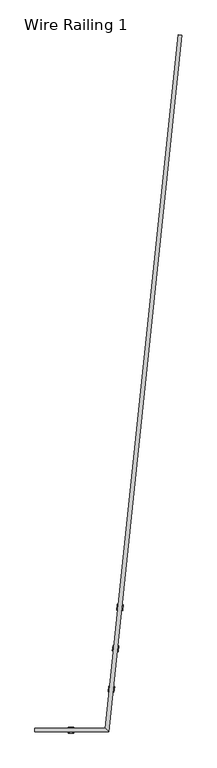
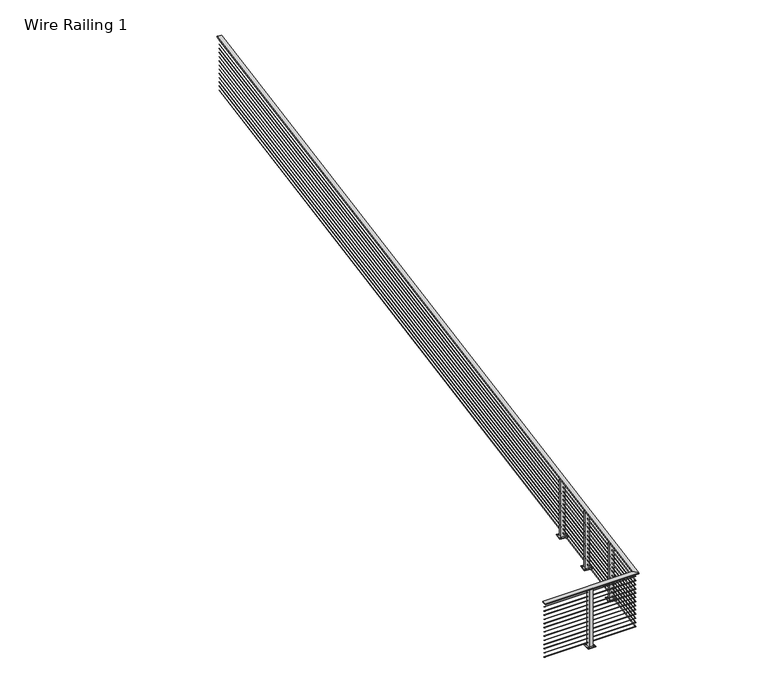
"""IFC4 building model written with IfcOpenShell, lengths in millimetres: railing geometry, Wire Railing 1."""

from ifc_helpers import new_model, si_unit, point, frame, frame_2d, origin, place, context, project, spatial, polyline, circle_curve, ellipse_curve, trimmed, segment, composite_curve, outline, extrude, faceted_brep, source, transform, mapped, element, save
from ifc_brep_helpers import plane_surface, cylinder_surface, advanced_brep


def wire_railing_1_9c637a7e(model_context):
    return source(origin(), model_context, "Body", "SolidModel", [
        faceted_brep([(32149.4090378, 25546.7031612, 267462.0), (32149.4090378, 25622.9031612, 267462.0), (32149.4090378, 25622.9031612, 267442.95), (32149.4090378, 25546.7031612, 267442.95), (33761.2935907, 25546.7031612, 267462.0), (33692.6828025, 25622.9031612, 267462.0), (33692.6828025, 25622.9031612, 267442.95), (33761.2935907, 25546.7031612, 267442.95), (35362.5021796, 40781.1852433, 267462.0), (35362.5021796, 40781.1852433, 267442.95), (35286.7196112, 40789.1503122, 267442.95), (35286.7196112, 40789.1503122, 267462.0)], [[[0, 1, 2, 3]], [[4, 5, 1, 0]], [[5, 6, 2, 1]], [[6, 7, 3, 2]], [[7, 4, 0, 3]], [[8, 9, 10, 11]], [[9, 8, 4, 7]], [[10, 9, 7, 6]], [[11, 10, 6, 5]], [[8, 11, 5, 4]]]),
        advanced_brep(
        [(32149.4090378, 25587.1844112, 267383.41875), (32149.4090378, 25582.4219112, 267383.41875), (33724.8441095, 25587.1844112, 267383.41875), (33729.1322837, 25582.4219112, 267383.41875), (35322.2426901, 40785.4166861, 267383.41875), (35326.9791007, 40784.9188693, 267383.41875)],
        [
            (0, 1, circle_curve(frame((32149.4090378, 25584.8031612, 267383.41875), z_axis=(-1.0, 0.0, 0.0), x_axis=(0.0, -1.0, 0.0)), 2.38125)),
            (1, 0, circle_curve(frame((32149.4090378, 25584.8031612, 267383.41875), z_axis=(-1.0, 0.0, 0.0), x_axis=(0.0, -1.0, 0.0)), 2.38125)),
            (2, 3, ellipse_curve(frame((33726.9881966, 25584.8031612, 267383.41875), z_axis=(-0.7431448254773928, -0.66913060635886, 0.0), x_axis=(0.6691306063588597, -0.7431448254773928, 0.0)), 3.2042879, 2.38125)),
            (3, 1),
            (0, 2),
            (3, 2, ellipse_curve(frame((33726.9881966, 25584.8031612, 267383.41875), z_axis=(-0.7431448254773928, -0.66913060635886, 0.0), x_axis=(0.6691306063588597, -0.7431448254773928, 0.0)), 3.2042879, 2.38125)),
            (4, 5, circle_curve(frame((35324.6108954, 40785.1677777, 267383.41875), z_axis=(0.10452846326764917, 0.9945218953682738, 0.0), x_axis=(0.9945218953682738, -0.10452846326764917, 0.0)), 2.38125)),
            (5, 4, circle_curve(frame((35324.6108954, 40785.1677777, 267383.41875), z_axis=(0.10452846326764917, 0.9945218953682738, 0.0), x_axis=(0.9945218953682738, -0.10452846326764917, 0.0)), 2.38125)),
            (4, 2),
            (3, 5),
        ],
        [
            plane_surface(frame((32149.4090378, 25584.8031612, 267385.8), z_axis=(-1.0, 0.0, 0.0), x_axis=(0.0, -1.0, 0.0))),
            cylinder_surface(frame((33726.9881966, 25584.8031612, 267383.41875), z_axis=(1.0, 0.0, 0.0), x_axis=(0.0, -1.0, 0.0)), 2.38125),
            plane_surface(frame((35324.6108954, 40785.1677777, 267385.8), z_axis=(0.10452846326764917, 0.9945218953682738, 0.0), x_axis=(0.9945218953682738, -0.10452846326764917, 0.0))),
            cylinder_surface(frame((35324.6108954, 40785.1677777, 267383.41875), z_axis=(0.10452846326764917, 0.9945218953682738, 0.0), x_axis=(0.9945218953682738, -0.10452846326764917, 0.0)), 2.38125),
        ],
        [
            (0, [[1, 2]]),
            (1, [[3, 4, -1, 5]]),
            (1, [[6, -5, -2, -4]]),
            (2, [[7, 8]]),
            (3, [[-7, 9, -6, 10]]),
            (3, [[-8, -10, -3, -9]]),
        ],
    ),
        advanced_brep(
        [(32149.4090378, 25587.1844112, 267307.21875), (32149.4090378, 25582.4219112, 267307.21875), (33724.8441095, 25587.1844112, 267307.21875), (33729.1322837, 25582.4219112, 267307.21875), (35322.2426901, 40785.4166861, 267307.21875), (35326.9791007, 40784.9188693, 267307.21875)],
        [
            (0, 1, circle_curve(frame((32149.4090378, 25584.8031612, 267307.21875), z_axis=(-1.0, 0.0, 0.0), x_axis=(0.0, -1.0, 0.0)), 2.38125)),
            (1, 0, circle_curve(frame((32149.4090378, 25584.8031612, 267307.21875), z_axis=(-1.0, 0.0, 0.0), x_axis=(0.0, -1.0, 0.0)), 2.38125)),
            (2, 3, ellipse_curve(frame((33726.9881966, 25584.8031612, 267307.21875), z_axis=(-0.7431448254773928, -0.66913060635886, 0.0), x_axis=(0.6691306063588597, -0.7431448254773928, 0.0)), 3.2042879, 2.38125)),
            (3, 1),
            (0, 2),
            (3, 2, ellipse_curve(frame((33726.9881966, 25584.8031612, 267307.21875), z_axis=(-0.7431448254773928, -0.66913060635886, 0.0), x_axis=(0.6691306063588597, -0.7431448254773928, 0.0)), 3.2042879, 2.38125)),
            (4, 5, circle_curve(frame((35324.6108954, 40785.1677777, 267307.21875), z_axis=(0.10452846326764917, 0.9945218953682738, 0.0), x_axis=(0.9945218953682738, -0.10452846326764917, 0.0)), 2.38125)),
            (5, 4, circle_curve(frame((35324.6108954, 40785.1677777, 267307.21875), z_axis=(0.10452846326764917, 0.9945218953682738, 0.0), x_axis=(0.9945218953682738, -0.10452846326764917, 0.0)), 2.38125)),
            (4, 2),
            (3, 5),
        ],
        [
            plane_surface(frame((32149.4090378, 25584.8031612, 267309.6), z_axis=(-1.0, 0.0, 0.0), x_axis=(0.0, -1.0, 0.0))),
            cylinder_surface(frame((33726.9881966, 25584.8031612, 267307.21875), z_axis=(1.0, 0.0, 0.0), x_axis=(0.0, -1.0, 0.0)), 2.38125),
            plane_surface(frame((35324.6108954, 40785.1677777, 267309.6), z_axis=(0.10452846326764917, 0.9945218953682738, 0.0), x_axis=(0.9945218953682738, -0.10452846326764917, 0.0))),
            cylinder_surface(frame((35324.6108954, 40785.1677777, 267307.21875), z_axis=(0.10452846326764917, 0.9945218953682738, 0.0), x_axis=(0.9945218953682738, -0.10452846326764917, 0.0)), 2.38125),
        ],
        [
            (0, [[1, 2]]),
            (1, [[3, 4, -1, 5]]),
            (1, [[6, -5, -2, -4]]),
            (2, [[7, 8]]),
            (3, [[-7, 9, -6, 10]]),
            (3, [[-8, -10, -3, -9]]),
        ],
    ),
        advanced_brep(
        [(32149.4090378, 25587.1844112, 267231.01875), (32149.4090378, 25582.4219112, 267231.01875), (33724.8441095, 25587.1844112, 267231.01875), (33729.1322837, 25582.4219112, 267231.01875), (35322.2426901, 40785.4166861, 267231.01875), (35326.9791007, 40784.9188693, 267231.01875)],
        [
            (0, 1, circle_curve(frame((32149.4090378, 25584.8031612, 267231.01875), z_axis=(-1.0, 0.0, 0.0), x_axis=(0.0, -1.0, 0.0)), 2.38125)),
            (1, 0, circle_curve(frame((32149.4090378, 25584.8031612, 267231.01875), z_axis=(-1.0, 0.0, 0.0), x_axis=(0.0, -1.0, 0.0)), 2.38125)),
            (2, 3, ellipse_curve(frame((33726.9881966, 25584.8031612, 267231.01875), z_axis=(-0.7431448254773928, -0.66913060635886, 0.0), x_axis=(0.6691306063588597, -0.7431448254773928, 0.0)), 3.2042879, 2.38125)),
            (3, 1),
            (0, 2),
            (3, 2, ellipse_curve(frame((33726.9881966, 25584.8031612, 267231.01875), z_axis=(-0.7431448254773928, -0.66913060635886, 0.0), x_axis=(0.6691306063588597, -0.7431448254773928, 0.0)), 3.2042879, 2.38125)),
            (4, 5, circle_curve(frame((35324.6108954, 40785.1677777, 267231.01875), z_axis=(0.10452846326764917, 0.9945218953682738, 0.0), x_axis=(0.9945218953682738, -0.10452846326764917, 0.0)), 2.38125)),
            (5, 4, circle_curve(frame((35324.6108954, 40785.1677777, 267231.01875), z_axis=(0.10452846326764917, 0.9945218953682738, 0.0), x_axis=(0.9945218953682738, -0.10452846326764917, 0.0)), 2.38125)),
            (4, 2),
            (3, 5),
        ],
        [
            plane_surface(frame((32149.4090378, 25584.8031612, 267233.4), z_axis=(-1.0, 0.0, 0.0), x_axis=(0.0, -1.0, 0.0))),
            cylinder_surface(frame((33726.9881966, 25584.8031612, 267231.01875), z_axis=(1.0, 0.0, 0.0), x_axis=(0.0, -1.0, 0.0)), 2.38125),
            plane_surface(frame((35324.6108954, 40785.1677777, 267233.4), z_axis=(0.10452846326764917, 0.9945218953682738, 0.0), x_axis=(0.9945218953682738, -0.10452846326764917, 0.0))),
            cylinder_surface(frame((35324.6108954, 40785.1677777, 267231.01875), z_axis=(0.10452846326764917, 0.9945218953682738, 0.0), x_axis=(0.9945218953682738, -0.10452846326764917, 0.0)), 2.38125),
        ],
        [
            (0, [[1, 2]]),
            (1, [[3, 4, -1, 5]]),
            (1, [[6, -5, -2, -4]]),
            (2, [[7, 8]]),
            (3, [[-7, 9, -6, 10]]),
            (3, [[-8, -10, -3, -9]]),
        ],
    ),
        advanced_brep(
        [(32149.4090378, 25587.1844112, 267154.81875), (32149.4090378, 25582.4219112, 267154.81875), (33724.8441095, 25587.1844112, 267154.81875), (33729.1322837, 25582.4219112, 267154.81875), (35322.2426901, 40785.4166861, 267154.81875), (35326.9791007, 40784.9188693, 267154.81875)],
        [
            (0, 1, circle_curve(frame((32149.4090378, 25584.8031612, 267154.81875), z_axis=(-1.0, 0.0, 0.0), x_axis=(0.0, -1.0, 0.0)), 2.38125)),
            (1, 0, circle_curve(frame((32149.4090378, 25584.8031612, 267154.81875), z_axis=(-1.0, 0.0, 0.0), x_axis=(0.0, -1.0, 0.0)), 2.38125)),
            (2, 3, ellipse_curve(frame((33726.9881966, 25584.8031612, 267154.81875), z_axis=(-0.7431448254773928, -0.66913060635886, 0.0), x_axis=(0.6691306063588597, -0.7431448254773928, 0.0)), 3.2042879, 2.38125)),
            (3, 1),
            (0, 2),
            (3, 2, ellipse_curve(frame((33726.9881966, 25584.8031612, 267154.81875), z_axis=(-0.7431448254773928, -0.66913060635886, 0.0), x_axis=(0.6691306063588597, -0.7431448254773928, 0.0)), 3.2042879, 2.38125)),
            (4, 5, circle_curve(frame((35324.6108954, 40785.1677777, 267154.81875), z_axis=(0.10452846326764917, 0.9945218953682738, 0.0), x_axis=(0.9945218953682738, -0.10452846326764917, 0.0)), 2.38125)),
            (5, 4, circle_curve(frame((35324.6108954, 40785.1677777, 267154.81875), z_axis=(0.10452846326764917, 0.9945218953682738, 0.0), x_axis=(0.9945218953682738, -0.10452846326764917, 0.0)), 2.38125)),
            (4, 2),
            (3, 5),
        ],
        [
            plane_surface(frame((32149.4090378, 25584.8031612, 267157.2), z_axis=(-1.0, 0.0, 0.0), x_axis=(0.0, -1.0, 0.0))),
            cylinder_surface(frame((33726.9881966, 25584.8031612, 267154.81875), z_axis=(1.0, 0.0, 0.0), x_axis=(0.0, -1.0, 0.0)), 2.38125),
            plane_surface(frame((35324.6108954, 40785.1677777, 267157.2), z_axis=(0.10452846326764917, 0.9945218953682738, 0.0), x_axis=(0.9945218953682738, -0.10452846326764917, 0.0))),
            cylinder_surface(frame((35324.6108954, 40785.1677777, 267154.81875), z_axis=(0.10452846326764917, 0.9945218953682738, 0.0), x_axis=(0.9945218953682738, -0.10452846326764917, 0.0)), 2.38125),
        ],
        [
            (0, [[1, 2]]),
            (1, [[3, 4, -1, 5]]),
            (1, [[6, -5, -2, -4]]),
            (2, [[7, 8]]),
            (3, [[-7, 9, -6, 10]]),
            (3, [[-8, -10, -3, -9]]),
        ],
    ),
        advanced_brep(
        [(32149.4090378, 25587.1844112, 267078.61875), (32149.4090378, 25582.4219112, 267078.61875), (33724.8441095, 25587.1844112, 267078.61875), (33729.1322837, 25582.4219112, 267078.61875), (35322.2426901, 40785.4166861, 267078.61875), (35326.9791007, 40784.9188693, 267078.61875)],
        [
            (0, 1, circle_curve(frame((32149.4090378, 25584.8031612, 267078.61875), z_axis=(-1.0, 0.0, 0.0), x_axis=(0.0, -1.0, 0.0)), 2.38125)),
            (1, 0, circle_curve(frame((32149.4090378, 25584.8031612, 267078.61875), z_axis=(-1.0, 0.0, 0.0), x_axis=(0.0, -1.0, 0.0)), 2.38125)),
            (2, 3, ellipse_curve(frame((33726.9881966, 25584.8031612, 267078.61875), z_axis=(-0.7431448254773928, -0.66913060635886, 0.0), x_axis=(0.6691306063588597, -0.7431448254773928, 0.0)), 3.2042879, 2.38125)),
            (3, 1),
            (0, 2),
            (3, 2, ellipse_curve(frame((33726.9881966, 25584.8031612, 267078.61875), z_axis=(-0.7431448254773928, -0.66913060635886, 0.0), x_axis=(0.6691306063588597, -0.7431448254773928, 0.0)), 3.2042879, 2.38125)),
            (4, 5, circle_curve(frame((35324.6108954, 40785.1677777, 267078.61875), z_axis=(0.10452846326764917, 0.9945218953682738, 0.0), x_axis=(0.9945218953682738, -0.10452846326764917, 0.0)), 2.38125)),
            (5, 4, circle_curve(frame((35324.6108954, 40785.1677777, 267078.61875), z_axis=(0.10452846326764917, 0.9945218953682738, 0.0), x_axis=(0.9945218953682738, -0.10452846326764917, 0.0)), 2.38125)),
            (4, 2),
            (3, 5),
        ],
        [
            plane_surface(frame((32149.4090378, 25584.8031612, 267081.0), z_axis=(-1.0, 0.0, 0.0), x_axis=(0.0, -1.0, 0.0))),
            cylinder_surface(frame((33726.9881966, 25584.8031612, 267078.61875), z_axis=(1.0, 0.0, 0.0), x_axis=(0.0, -1.0, 0.0)), 2.38125),
            plane_surface(frame((35324.6108954, 40785.1677777, 267081.0), z_axis=(0.10452846326764917, 0.9945218953682738, 0.0), x_axis=(0.9945218953682738, -0.10452846326764917, 0.0))),
            cylinder_surface(frame((35324.6108954, 40785.1677777, 267078.61875), z_axis=(0.10452846326764917, 0.9945218953682738, 0.0), x_axis=(0.9945218953682738, -0.10452846326764917, 0.0)), 2.38125),
        ],
        [
            (0, [[1, 2]]),
            (1, [[3, 4, -1, 5]]),
            (1, [[6, -5, -2, -4]]),
            (2, [[7, 8]]),
            (3, [[-7, 9, -6, 10]]),
            (3, [[-8, -10, -3, -9]]),
        ],
    ),
        advanced_brep(
        [(32149.4090378, 25587.1844112, 267002.41875), (32149.4090378, 25582.4219112, 267002.41875), (33724.8441095, 25587.1844112, 267002.41875), (33729.1322837, 25582.4219112, 267002.41875), (35322.2426901, 40785.4166861, 267002.41875), (35326.9791007, 40784.9188693, 267002.41875)],
        [
            (0, 1, circle_curve(frame((32149.4090378, 25584.8031612, 267002.41875), z_axis=(-1.0, 0.0, 0.0), x_axis=(0.0, -1.0, 0.0)), 2.38125)),
            (1, 0, circle_curve(frame((32149.4090378, 25584.8031612, 267002.41875), z_axis=(-1.0, 0.0, 0.0), x_axis=(0.0, -1.0, 0.0)), 2.38125)),
            (2, 3, ellipse_curve(frame((33726.9881966, 25584.8031612, 267002.41875), z_axis=(-0.7431448254773928, -0.66913060635886, 0.0), x_axis=(0.6691306063588597, -0.7431448254773928, 0.0)), 3.2042879, 2.38125)),
            (3, 1),
            (0, 2),
            (3, 2, ellipse_curve(frame((33726.9881966, 25584.8031612, 267002.41875), z_axis=(-0.7431448254773928, -0.66913060635886, 0.0), x_axis=(0.6691306063588597, -0.7431448254773928, 0.0)), 3.2042879, 2.38125)),
            (4, 5, circle_curve(frame((35324.6108954, 40785.1677777, 267002.41875), z_axis=(0.10452846326764917, 0.9945218953682738, 0.0), x_axis=(0.9945218953682738, -0.10452846326764917, 0.0)), 2.38125)),
            (5, 4, circle_curve(frame((35324.6108954, 40785.1677777, 267002.41875), z_axis=(0.10452846326764917, 0.9945218953682738, 0.0), x_axis=(0.9945218953682738, -0.10452846326764917, 0.0)), 2.38125)),
            (4, 2),
            (3, 5),
        ],
        [
            plane_surface(frame((32149.4090378, 25584.8031612, 267004.8), z_axis=(-1.0, 0.0, 0.0), x_axis=(0.0, -1.0, 0.0))),
            cylinder_surface(frame((33726.9881966, 25584.8031612, 267002.41875), z_axis=(1.0, 0.0, 0.0), x_axis=(0.0, -1.0, 0.0)), 2.38125),
            plane_surface(frame((35324.6108954, 40785.1677777, 267004.8), z_axis=(0.10452846326764917, 0.9945218953682738, 0.0), x_axis=(0.9945218953682738, -0.10452846326764917, 0.0))),
            cylinder_surface(frame((35324.6108954, 40785.1677777, 267002.41875), z_axis=(0.10452846326764917, 0.9945218953682738, 0.0), x_axis=(0.9945218953682738, -0.10452846326764917, 0.0)), 2.38125),
        ],
        [
            (0, [[1, 2]]),
            (1, [[3, 4, -1, 5]]),
            (1, [[6, -5, -2, -4]]),
            (2, [[7, 8]]),
            (3, [[-7, 9, -6, 10]]),
            (3, [[-8, -10, -3, -9]]),
        ],
    ),
        advanced_brep(
        [(32149.4090378, 25587.1844112, 266926.21875), (32149.4090378, 25582.4219112, 266926.21875), (33724.8441095, 25587.1844112, 266926.21875), (33729.1322837, 25582.4219112, 266926.21875), (35322.2426901, 40785.4166861, 266926.21875), (35326.9791007, 40784.9188693, 266926.21875)],
        [
            (0, 1, circle_curve(frame((32149.4090378, 25584.8031612, 266926.21875), z_axis=(-1.0, 0.0, 0.0), x_axis=(0.0, -1.0, 0.0)), 2.38125)),
            (1, 0, circle_curve(frame((32149.4090378, 25584.8031612, 266926.21875), z_axis=(-1.0, 0.0, 0.0), x_axis=(0.0, -1.0, 0.0)), 2.38125)),
            (2, 3, ellipse_curve(frame((33726.9881966, 25584.8031612, 266926.21875), z_axis=(-0.7431448254773928, -0.66913060635886, 0.0), x_axis=(0.6691306063588597, -0.7431448254773928, 0.0)), 3.2042879, 2.38125)),
            (3, 1),
            (0, 2),
            (3, 2, ellipse_curve(frame((33726.9881966, 25584.8031612, 266926.21875), z_axis=(-0.7431448254773928, -0.66913060635886, 0.0), x_axis=(0.6691306063588597, -0.7431448254773928, 0.0)), 3.2042879, 2.38125)),
            (4, 5, circle_curve(frame((35324.6108954, 40785.1677777, 266926.21875), z_axis=(0.10452846326764917, 0.9945218953682738, 0.0), x_axis=(0.9945218953682738, -0.10452846326764917, 0.0)), 2.38125)),
            (5, 4, circle_curve(frame((35324.6108954, 40785.1677777, 266926.21875), z_axis=(0.10452846326764917, 0.9945218953682738, 0.0), x_axis=(0.9945218953682738, -0.10452846326764917, 0.0)), 2.38125)),
            (4, 2),
            (3, 5),
        ],
        [
            plane_surface(frame((32149.4090378, 25584.8031612, 266928.6), z_axis=(-1.0, 0.0, 0.0), x_axis=(0.0, -1.0, 0.0))),
            cylinder_surface(frame((33726.9881966, 25584.8031612, 266926.21875), z_axis=(1.0, 0.0, 0.0), x_axis=(0.0, -1.0, 0.0)), 2.38125),
            plane_surface(frame((35324.6108954, 40785.1677777, 266928.6), z_axis=(0.10452846326764917, 0.9945218953682738, 0.0), x_axis=(0.9945218953682738, -0.10452846326764917, 0.0))),
            cylinder_surface(frame((35324.6108954, 40785.1677777, 266926.21875), z_axis=(0.10452846326764917, 0.9945218953682738, 0.0), x_axis=(0.9945218953682738, -0.10452846326764917, 0.0)), 2.38125),
        ],
        [
            (0, [[1, 2]]),
            (1, [[3, 4, -1, 5]]),
            (1, [[6, -5, -2, -4]]),
            (2, [[7, 8]]),
            (3, [[-7, 9, -6, 10]]),
            (3, [[-8, -10, -3, -9]]),
        ],
    ),
        advanced_brep(
        [(32149.4090378, 25587.1844112, 266850.01875), (32149.4090378, 25582.4219112, 266850.01875), (33724.8441095, 25587.1844112, 266850.01875), (33729.1322837, 25582.4219112, 266850.01875), (35322.2426901, 40785.4166861, 266850.01875), (35326.9791007, 40784.9188693, 266850.01875)],
        [
            (0, 1, circle_curve(frame((32149.4090378, 25584.8031612, 266850.01875), z_axis=(-1.0, 0.0, 0.0), x_axis=(0.0, -1.0, 0.0)), 2.38125)),
            (1, 0, circle_curve(frame((32149.4090378, 25584.8031612, 266850.01875), z_axis=(-1.0, 0.0, 0.0), x_axis=(0.0, -1.0, 0.0)), 2.38125)),
            (2, 3, ellipse_curve(frame((33726.9881966, 25584.8031612, 266850.01875), z_axis=(-0.7431448254773928, -0.66913060635886, 0.0), x_axis=(0.6691306063588597, -0.7431448254773928, 0.0)), 3.2042879, 2.38125)),
            (3, 1),
            (0, 2),
            (3, 2, ellipse_curve(frame((33726.9881966, 25584.8031612, 266850.01875), z_axis=(-0.7431448254773928, -0.66913060635886, 0.0), x_axis=(0.6691306063588597, -0.7431448254773928, 0.0)), 3.2042879, 2.38125)),
            (4, 5, circle_curve(frame((35324.6108954, 40785.1677777, 266850.01875), z_axis=(0.10452846326764917, 0.9945218953682738, 0.0), x_axis=(0.9945218953682738, -0.10452846326764917, 0.0)), 2.38125)),
            (5, 4, circle_curve(frame((35324.6108954, 40785.1677777, 266850.01875), z_axis=(0.10452846326764917, 0.9945218953682738, 0.0), x_axis=(0.9945218953682738, -0.10452846326764917, 0.0)), 2.38125)),
            (4, 2),
            (3, 5),
        ],
        [
            plane_surface(frame((32149.4090378, 25584.8031612, 266852.4), z_axis=(-1.0, 0.0, 0.0), x_axis=(0.0, -1.0, 0.0))),
            cylinder_surface(frame((33726.9881966, 25584.8031612, 266850.01875), z_axis=(1.0, 0.0, 0.0), x_axis=(0.0, -1.0, 0.0)), 2.38125),
            plane_surface(frame((35324.6108954, 40785.1677777, 266852.4), z_axis=(0.10452846326764917, 0.9945218953682738, 0.0), x_axis=(0.9945218953682738, -0.10452846326764917, 0.0))),
            cylinder_surface(frame((35324.6108954, 40785.1677777, 266850.01875), z_axis=(0.10452846326764917, 0.9945218953682738, 0.0), x_axis=(0.9945218953682738, -0.10452846326764917, 0.0)), 2.38125),
        ],
        [
            (0, [[1, 2]]),
            (1, [[3, 4, -1, 5]]),
            (1, [[6, -5, -2, -4]]),
            (2, [[7, 8]]),
            (3, [[-7, 9, -6, 10]]),
            (3, [[-8, -10, -3, -9]]),
        ],
    ),
        advanced_brep(
        [(32149.4090378, 25587.1844112, 266773.81875), (32149.4090378, 25582.4219112, 266773.81875), (33724.8441095, 25587.1844112, 266773.81875), (33729.1322837, 25582.4219112, 266773.81875), (35322.2426901, 40785.4166861, 266773.81875), (35326.9791007, 40784.9188693, 266773.81875)],
        [
            (0, 1, circle_curve(frame((32149.4090378, 25584.8031612, 266773.81875), z_axis=(-1.0, 0.0, 0.0), x_axis=(0.0, -1.0, 0.0)), 2.38125)),
            (1, 0, circle_curve(frame((32149.4090378, 25584.8031612, 266773.81875), z_axis=(-1.0, 0.0, 0.0), x_axis=(0.0, -1.0, 0.0)), 2.38125)),
            (2, 3, ellipse_curve(frame((33726.9881966, 25584.8031612, 266773.81875), z_axis=(-0.7431448254773928, -0.66913060635886, 0.0), x_axis=(0.6691306063588597, -0.7431448254773928, 0.0)), 3.2042879, 2.38125)),
            (3, 1),
            (0, 2),
            (3, 2, ellipse_curve(frame((33726.9881966, 25584.8031612, 266773.81875), z_axis=(-0.7431448254773928, -0.66913060635886, 0.0), x_axis=(0.6691306063588597, -0.7431448254773928, 0.0)), 3.2042879, 2.38125)),
            (4, 5, circle_curve(frame((35324.6108954, 40785.1677777, 266773.81875), z_axis=(0.10452846326764917, 0.9945218953682738, 0.0), x_axis=(0.9945218953682738, -0.10452846326764917, 0.0)), 2.38125)),
            (5, 4, circle_curve(frame((35324.6108954, 40785.1677777, 266773.81875), z_axis=(0.10452846326764917, 0.9945218953682738, 0.0), x_axis=(0.9945218953682738, -0.10452846326764917, 0.0)), 2.38125)),
            (4, 2),
            (3, 5),
        ],
        [
            plane_surface(frame((32149.4090378, 25584.8031612, 266776.2), z_axis=(-1.0, 0.0, 0.0), x_axis=(0.0, -1.0, 0.0))),
            cylinder_surface(frame((33726.9881966, 25584.8031612, 266773.81875), z_axis=(1.0, 0.0, 0.0), x_axis=(0.0, -1.0, 0.0)), 2.38125),
            plane_surface(frame((35324.6108954, 40785.1677777, 266776.2), z_axis=(0.10452846326764917, 0.9945218953682738, 0.0), x_axis=(0.9945218953682738, -0.10452846326764917, 0.0))),
            cylinder_surface(frame((35324.6108954, 40785.1677777, 266773.81875), z_axis=(0.10452846326764917, 0.9945218953682738, 0.0), x_axis=(0.9945218953682738, -0.10452846326764917, 0.0)), 2.38125),
        ],
        [
            (0, [[1, 2]]),
            (1, [[3, 4, -1, 5]]),
            (1, [[6, -5, -2, -4]]),
            (2, [[7, 8]]),
            (3, [[-7, 9, -6, 10]]),
            (3, [[-8, -10, -3, -9]]),
        ],
    ),
        advanced_brep(
        [(32149.4090378, 25587.1844112, 266697.61875), (32149.4090378, 25582.4219112, 266697.61875), (33724.8441095, 25587.1844112, 266697.61875), (33729.1322837, 25582.4219112, 266697.61875), (35322.2426901, 40785.4166861, 266697.61875), (35326.9791007, 40784.9188693, 266697.61875)],
        [
            (0, 1, circle_curve(frame((32149.4090378, 25584.8031612, 266697.61875), z_axis=(-1.0, 0.0, 0.0), x_axis=(0.0, -1.0, 0.0)), 2.38125)),
            (1, 0, circle_curve(frame((32149.4090378, 25584.8031612, 266697.61875), z_axis=(-1.0, 0.0, 0.0), x_axis=(0.0, -1.0, 0.0)), 2.38125)),
            (2, 3, ellipse_curve(frame((33726.9881966, 25584.8031612, 266697.61875), z_axis=(-0.7431448254773928, -0.66913060635886, 0.0), x_axis=(0.6691306063588597, -0.7431448254773928, 0.0)), 3.2042879, 2.38125)),
            (3, 1),
            (0, 2),
            (3, 2, ellipse_curve(frame((33726.9881966, 25584.8031612, 266697.61875), z_axis=(-0.7431448254773928, -0.66913060635886, 0.0), x_axis=(0.6691306063588597, -0.7431448254773928, 0.0)), 3.2042879, 2.38125)),
            (4, 5, circle_curve(frame((35324.6108954, 40785.1677777, 266697.61875), z_axis=(0.10452846326764917, 0.9945218953682738, 0.0), x_axis=(0.9945218953682738, -0.10452846326764917, 0.0)), 2.38125)),
            (5, 4, circle_curve(frame((35324.6108954, 40785.1677777, 266697.61875), z_axis=(0.10452846326764917, 0.9945218953682738, 0.0), x_axis=(0.9945218953682738, -0.10452846326764917, 0.0)), 2.38125)),
            (4, 2),
            (3, 5),
        ],
        [
            plane_surface(frame((32149.4090378, 25584.8031612, 266700.0), z_axis=(-1.0, 0.0, 0.0), x_axis=(0.0, -1.0, 0.0))),
            cylinder_surface(frame((33726.9881966, 25584.8031612, 266697.61875), z_axis=(1.0, 0.0, 0.0), x_axis=(0.0, -1.0, 0.0)), 2.38125),
            plane_surface(frame((35324.6108954, 40785.1677777, 266700.0), z_axis=(0.10452846326764917, 0.9945218953682738, 0.0), x_axis=(0.9945218953682738, -0.10452846326764917, 0.0))),
            cylinder_surface(frame((35324.6108954, 40785.1677777, 266697.61875), z_axis=(0.10452846326764917, 0.9945218953682738, 0.0), x_axis=(0.9945218953682738, -0.10452846326764917, 0.0)), 2.38125),
        ],
        [
            (0, [[1, 2]]),
            (1, [[3, 4, -1, 5]]),
            (1, [[6, -5, -2, -4]]),
            (2, [[7, 8]]),
            (3, [[-7, 9, -6, 10]]),
            (3, [[-8, -10, -3, -9]]),
        ],
    ),
        advanced_brep(
        [(32149.4090378, 25587.1844112, 266621.41875), (32149.4090378, 25582.4219112, 266621.41875), (33724.8441095, 25587.1844112, 266621.41875), (33729.1322837, 25582.4219112, 266621.41875), (35322.2426901, 40785.4166861, 266621.41875), (35326.9791007, 40784.9188693, 266621.41875)],
        [
            (0, 1, circle_curve(frame((32149.4090378, 25584.8031612, 266621.41875), z_axis=(-1.0, 0.0, 0.0), x_axis=(0.0, -1.0, 0.0)), 2.38125)),
            (1, 0, circle_curve(frame((32149.4090378, 25584.8031612, 266621.41875), z_axis=(-1.0, 0.0, 0.0), x_axis=(0.0, -1.0, 0.0)), 2.38125)),
            (2, 3, ellipse_curve(frame((33726.9881966, 25584.8031612, 266621.41875), z_axis=(-0.7431448254773928, -0.66913060635886, 0.0), x_axis=(0.6691306063588597, -0.7431448254773928, 0.0)), 3.2042879, 2.38125)),
            (3, 1),
            (0, 2),
            (3, 2, ellipse_curve(frame((33726.9881966, 25584.8031612, 266621.41875), z_axis=(-0.7431448254773928, -0.66913060635886, 0.0), x_axis=(0.6691306063588597, -0.7431448254773928, 0.0)), 3.2042879, 2.38125)),
            (4, 5, circle_curve(frame((35324.6108954, 40785.1677777, 266621.41875), z_axis=(0.10452846326764917, 0.9945218953682738, 0.0), x_axis=(0.9945218953682738, -0.10452846326764917, 0.0)), 2.38125)),
            (5, 4, circle_curve(frame((35324.6108954, 40785.1677777, 266621.41875), z_axis=(0.10452846326764917, 0.9945218953682738, 0.0), x_axis=(0.9945218953682738, -0.10452846326764917, 0.0)), 2.38125)),
            (4, 2),
            (3, 5),
        ],
        [
            plane_surface(frame((32149.4090378, 25584.8031612, 266623.8), z_axis=(-1.0, 0.0, 0.0), x_axis=(0.0, -1.0, 0.0))),
            cylinder_surface(frame((33726.9881966, 25584.8031612, 266621.41875), z_axis=(1.0, 0.0, 0.0), x_axis=(0.0, -1.0, 0.0)), 2.38125),
            plane_surface(frame((35324.6108954, 40785.1677777, 266623.8), z_axis=(0.10452846326764917, 0.9945218953682738, 0.0), x_axis=(0.9945218953682738, -0.10452846326764917, 0.0))),
            cylinder_surface(frame((35324.6108954, 40785.1677777, 266621.41875), z_axis=(0.10452846326764917, 0.9945218953682738, 0.0), x_axis=(0.9945218953682738, -0.10452846326764917, 0.0)), 2.38125),
        ],
        [
            (0, [[1, 2]]),
            (1, [[3, 4, -1, 5]]),
            (1, [[6, -5, -2, -4]]),
            (2, [[7, 8]]),
            (3, [[-7, 9, -6, 10]]),
            (3, [[-8, -10, -3, -9]]),
        ],
    ),
        advanced_brep(
        [(32149.4090378, 25587.1844112, 266545.21875), (32149.4090378, 25582.4219112, 266545.21875), (33724.8441095, 25587.1844112, 266545.21875), (33729.1322837, 25582.4219112, 266545.21875), (35322.2426901, 40785.4166861, 266545.21875), (35326.9791007, 40784.9188693, 266545.21875)],
        [
            (0, 1, circle_curve(frame((32149.4090378, 25584.8031612, 266545.21875), z_axis=(-1.0, 0.0, 0.0), x_axis=(0.0, -1.0, 0.0)), 2.38125)),
            (1, 0, circle_curve(frame((32149.4090378, 25584.8031612, 266545.21875), z_axis=(-1.0, 0.0, 0.0), x_axis=(0.0, -1.0, 0.0)), 2.38125)),
            (2, 3, ellipse_curve(frame((33726.9881966, 25584.8031612, 266545.21875), z_axis=(-0.7431448254773928, -0.66913060635886, 0.0), x_axis=(0.6691306063588597, -0.7431448254773928, 0.0)), 3.2042879, 2.38125)),
            (3, 1),
            (0, 2),
            (3, 2, ellipse_curve(frame((33726.9881966, 25584.8031612, 266545.21875), z_axis=(-0.7431448254773928, -0.66913060635886, 0.0), x_axis=(0.6691306063588597, -0.7431448254773928, 0.0)), 3.2042879, 2.38125)),
            (4, 5, circle_curve(frame((35324.6108954, 40785.1677777, 266545.21875), z_axis=(0.10452846326764917, 0.9945218953682738, 0.0), x_axis=(0.9945218953682738, -0.10452846326764917, 0.0)), 2.38125)),
            (5, 4, circle_curve(frame((35324.6108954, 40785.1677777, 266545.21875), z_axis=(0.10452846326764917, 0.9945218953682738, 0.0), x_axis=(0.9945218953682738, -0.10452846326764917, 0.0)), 2.38125)),
            (4, 2),
            (3, 5),
        ],
        [
            plane_surface(frame((32149.4090378, 25584.8031612, 266547.6), z_axis=(-1.0, 0.0, 0.0), x_axis=(0.0, -1.0, 0.0))),
            cylinder_surface(frame((33726.9881966, 25584.8031612, 266545.21875), z_axis=(1.0, 0.0, 0.0), x_axis=(0.0, -1.0, 0.0)), 2.38125),
            plane_surface(frame((35324.6108954, 40785.1677777, 266547.6), z_axis=(0.10452846326764917, 0.9945218953682738, 0.0), x_axis=(0.9945218953682738, -0.10452846326764917, 0.0))),
            cylinder_surface(frame((35324.6108954, 40785.1677777, 266545.21875), z_axis=(0.10452846326764917, 0.9945218953682738, 0.0), x_axis=(0.9945218953682738, -0.10452846326764917, 0.0)), 2.38125),
        ],
        [
            (0, [[1, 2]]),
            (1, [[3, 4, -1, 5]]),
            (1, [[6, -5, -2, -4]]),
            (2, [[7, 8]]),
            (3, [[-7, 9, -6, 10]]),
            (3, [[-8, -10, -3, -9]]),
        ],
    ),
        advanced_brep(
        [(32149.4090378, 25587.1844112, 266469.01875), (32149.4090378, 25582.4219112, 266469.01875), (33724.8441095, 25587.1844112, 266469.01875), (33729.1322837, 25582.4219112, 266469.01875), (35322.2426901, 40785.4166861, 266469.01875), (35326.9791007, 40784.9188693, 266469.01875)],
        [
            (0, 1, circle_curve(frame((32149.4090378, 25584.8031612, 266469.01875), z_axis=(-1.0, 0.0, 0.0), x_axis=(0.0, -1.0, 0.0)), 2.38125)),
            (1, 0, circle_curve(frame((32149.4090378, 25584.8031612, 266469.01875), z_axis=(-1.0, 0.0, 0.0), x_axis=(0.0, -1.0, 0.0)), 2.38125)),
            (2, 3, ellipse_curve(frame((33726.9881966, 25584.8031612, 266469.01875), z_axis=(-0.7431448254773928, -0.66913060635886, 0.0), x_axis=(0.6691306063588597, -0.7431448254773928, 0.0)), 3.2042879, 2.38125)),
            (3, 1),
            (0, 2),
            (3, 2, ellipse_curve(frame((33726.9881966, 25584.8031612, 266469.01875), z_axis=(-0.7431448254773928, -0.66913060635886, 0.0), x_axis=(0.6691306063588597, -0.7431448254773928, 0.0)), 3.2042879, 2.38125)),
            (4, 5, circle_curve(frame((35324.6108954, 40785.1677777, 266469.01875), z_axis=(0.10452846326764917, 0.9945218953682738, 0.0), x_axis=(0.9945218953682738, -0.10452846326764917, 0.0)), 2.38125)),
            (5, 4, circle_curve(frame((35324.6108954, 40785.1677777, 266469.01875), z_axis=(0.10452846326764917, 0.9945218953682738, 0.0), x_axis=(0.9945218953682738, -0.10452846326764917, 0.0)), 2.38125)),
            (4, 2),
            (3, 5),
        ],
        [
            plane_surface(frame((32149.4090378, 25584.8031612, 266471.4), z_axis=(-1.0, 0.0, 0.0), x_axis=(0.0, -1.0, 0.0))),
            cylinder_surface(frame((33726.9881966, 25584.8031612, 266469.01875), z_axis=(1.0, 0.0, 0.0), x_axis=(0.0, -1.0, 0.0)), 2.38125),
            plane_surface(frame((35324.6108954, 40785.1677777, 266471.4), z_axis=(0.10452846326764917, 0.9945218953682738, 0.0), x_axis=(0.9945218953682738, -0.10452846326764917, 0.0))),
            cylinder_surface(frame((35324.6108954, 40785.1677777, 266469.01875), z_axis=(0.10452846326764917, 0.9945218953682738, 0.0), x_axis=(0.9945218953682738, -0.10452846326764917, 0.0)), 2.38125),
        ],
        [
            (0, [[1, 2]]),
            (1, [[3, 4, -1, 5]]),
            (1, [[6, -5, -2, -4]]),
            (2, [[7, 8]]),
            (3, [[-7, 9, -6, 10]]),
            (3, [[-8, -10, -3, -9]]),
        ],
    ),
        extrude(outline(composite_curve([segment(trimmed(circle_curve(frame_2d((32982.6486172, 25540.3531612)), 6.35), [point((32982.6486172, 25534.0031612))], [point((32982.6486172, 25546.7031612))], False, "CARTESIAN"), True, "CONTINUOUS"), segment(trimmed(circle_curve(frame_2d((32982.6486172, 25540.3531612)), 6.35), [point((32982.6486172, 25546.7031612))], [point((32982.6486172, 25534.0031612))], False, "CARTESIAN"), True, "CONTINUOUS")], self_intersect=False)), frame((0.0, 0.0, 266395.2), z_axis=(0.0, 0.0, 1.0), x_axis=(1.0, 0.0, 0.0)), (0.0, 0.0, 1.0), 12.7),
        extrude(outline(composite_curve([segment(trimmed(circle_curve(frame_2d((32982.6486172, 25629.2531612)), 6.35), [point((32982.6486172, 25622.9031612))], [point((32982.6486172, 25635.6031612))], False, "CARTESIAN"), True, "CONTINUOUS"), segment(trimmed(circle_curve(frame_2d((32982.6486172, 25629.2531612)), 6.35), [point((32982.6486172, 25635.6031612))], [point((32982.6486172, 25622.9031612))], False, "CARTESIAN"), True, "CONTINUOUS")], self_intersect=False)), frame((0.0, 0.0, 266395.2), z_axis=(0.0, 0.0, 1.0), x_axis=(1.0, 0.0, 0.0)), (0.0, 0.0, 1.0), 12.7),
        extrude(outline(composite_curve([segment(trimmed(circle_curve(frame_2d((32893.7486172, 25540.3531612)), 6.35), [point((32893.7486172, 25534.0031612))], [point((32893.7486172, 25546.7031612))], False, "CARTESIAN"), True, "CONTINUOUS"), segment(trimmed(circle_curve(frame_2d((32893.7486172, 25540.3531612)), 6.35), [point((32893.7486172, 25546.7031612))], [point((32893.7486172, 25534.0031612))], False, "CARTESIAN"), True, "CONTINUOUS")], self_intersect=False)), frame((0.0, 0.0, 266395.2), z_axis=(0.0, 0.0, 1.0), x_axis=(1.0, 0.0, 0.0)), (0.0, 0.0, 1.0), 12.7),
        extrude(outline(composite_curve([segment(trimmed(circle_curve(frame_2d((32893.7486172, 25629.2531612)), 6.35), [point((32893.7486172, 25622.9031612))], [point((32893.7486172, 25635.6031612))], False, "CARTESIAN"), True, "CONTINUOUS"), segment(trimmed(circle_curve(frame_2d((32893.7486172, 25629.2531612)), 6.35), [point((32893.7486172, 25635.6031612))], [point((32893.7486172, 25622.9031612))], False, "CARTESIAN"), True, "CONTINUOUS")], self_intersect=False)), frame((0.0, 0.0, 266395.2), z_axis=(0.0, 0.0, 1.0), x_axis=(1.0, 0.0, 0.0)), (0.0, 0.0, 1.0), 12.7),
        extrude(outline(polyline([(33001.6986172, 25648.3031612), (33001.6986172, 25521.3031612), (32874.6986172, 25521.3031612), (32874.6986172, 25648.3031612), (33001.6986172, 25648.3031612)])), frame((0.0, 0.0, 266395.2), z_axis=(0.0, 0.0, 1.0), x_axis=(1.0, 0.0, 0.0)), (0.0, 0.0, 1.0), 6.35),
        extrude(outline(polyline([(32968.3611172, 25614.9656612), (32968.3611172, 25554.6406612), (32908.0361172, 25554.6406612), (32908.0361172, 25614.9656612), (32968.3611172, 25614.9656612)]), holes=[polyline([(32962.0111172, 25608.6156612), (32914.3861172, 25608.6156612), (32914.3861172, 25560.9906612), (32962.0111172, 25560.9906612), (32962.0111172, 25608.6156612)])]), frame((0.0, 0.0, 266395.2), z_axis=(0.0, 0.0, 1.0), x_axis=(1.0, 0.0, 0.0)), (0.0, 0.0, 1.0), 1047.75),
        extrude(outline(composite_curve([segment(trimmed(circle_curve(frame_2d((33869.8187909, 26518.5024643)), 6.35), [point((33876.1340049, 26517.8387086))], [point((33863.5035768, 26519.1662201))], False, "CARTESIAN"), True, "CONTINUOUS"), segment(trimmed(circle_curve(frame_2d((33869.8187909, 26518.5024643)), 6.35), [point((33863.5035768, 26519.1662201))], [point((33876.1340049, 26517.8387086))], False, "CARTESIAN"), True, "CONTINUOUS")], self_intersect=False)), frame((0.0, 0.0, 266395.2), z_axis=(0.0, 0.0, 1.0), x_axis=(1.0, 0.0, 0.0)), (0.0, 0.0, 1.0), 12.7),
        extrude(outline(composite_curve([segment(trimmed(circle_curve(frame_2d((33781.4057944, 26527.7950447)), 6.35), [point((33787.7210084, 26527.131289))], [point((33775.0905803, 26528.4588005))], False, "CARTESIAN"), True, "CONTINUOUS"), segment(trimmed(circle_curve(frame_2d((33781.4057944, 26527.7950447)), 6.35), [point((33775.0905803, 26528.4588005))], [point((33787.7210084, 26527.131289))], False, "CARTESIAN"), True, "CONTINUOUS")], self_intersect=False)), frame((0.0, 0.0, 266395.2), z_axis=(0.0, 0.0, 1.0), x_axis=(1.0, 0.0, 0.0)), (0.0, 0.0, 1.0), 12.7),
        extrude(outline(composite_curve([segment(trimmed(circle_curve(frame_2d((33860.5262105, 26430.0894678)), 6.35), [point((33866.8414245, 26429.4257121))], [point((33854.2109964, 26430.7532236))], False, "CARTESIAN"), True, "CONTINUOUS"), segment(trimmed(circle_curve(frame_2d((33860.5262105, 26430.0894678)), 6.35), [point((33854.2109964, 26430.7532236))], [point((33866.8414245, 26429.4257121))], False, "CARTESIAN"), True, "CONTINUOUS")], self_intersect=False)), frame((0.0, 0.0, 266395.2), z_axis=(0.0, 0.0, 1.0), x_axis=(1.0, 0.0, 0.0)), (0.0, 0.0, 1.0), 12.7),
        extrude(outline(composite_curve([segment(trimmed(circle_curve(frame_2d((33772.113214, 26439.3820482)), 6.35), [point((33778.428428, 26438.7182925))], [point((33765.7979999, 26440.045804))], False, "CARTESIAN"), True, "CONTINUOUS"), segment(trimmed(circle_curve(frame_2d((33772.113214, 26439.3820482)), 6.35), [point((33765.7979999, 26440.045804))], [point((33778.428428, 26438.7182925))], False, "CARTESIAN"), True, "CONTINUOUS")], self_intersect=False)), frame((0.0, 0.0, 266395.2), z_axis=(0.0, 0.0, 1.0), x_axis=(1.0, 0.0, 0.0)), (0.0, 0.0, 1.0), 12.7),
        extrude(outline(polyline([(33764.4514195, 26548.7319541), (33890.7557002, 26535.4568392), (33877.4805854, 26409.1525585), (33751.1763046, 26422.4276733), (33764.4514195, 26548.7319541)])), frame((0.0, 0.0, 266395.2), z_axis=(0.0, 0.0, 1.0), x_axis=(1.0, 0.0, 0.0)), (0.0, 0.0, 1.0), 6.35),
        extrude(outline(polyline([(33794.1215755, 26512.0923627), (33854.1161089, 26505.7866832), (33847.8104293, 26445.7921498), (33787.815896, 26452.0978294), (33794.1215755, 26512.0923627)]), holes=[polyline([(33799.7730338, 26505.113393), (33794.7948658, 26457.7492877), (33842.158971, 26452.7711196), (33847.1371391, 26500.1352249), (33799.7730338, 26505.113393)])]), frame((0.0, 0.0, 266395.2), z_axis=(0.0, 0.0, 1.0), x_axis=(1.0, 0.0, 0.0)), (0.0, 0.0, 1.0), 1047.75),
        extrude(outline(composite_curve([segment(trimmed(circle_curve(frame_2d((33963.7965967, 27412.6415594)), 6.35), [point((33970.1118107, 27411.9778037))], [point((33957.4813826, 27413.3053152))], False, "CARTESIAN"), True, "CONTINUOUS"), segment(trimmed(circle_curve(frame_2d((33963.7965967, 27412.6415594)), 6.35), [point((33957.4813826, 27413.3053152))], [point((33970.1118107, 27411.9778037))], False, "CARTESIAN"), True, "CONTINUOUS")], self_intersect=False)), frame((0.0, 0.0, 266395.2), z_axis=(0.0, 0.0, 1.0), x_axis=(1.0, 0.0, 0.0)), (0.0, 0.0, 1.0), 12.7),
        extrude(outline(composite_curve([segment(trimmed(circle_curve(frame_2d((33875.3836002, 27421.9341398)), 6.35), [point((33881.6988142, 27421.2703841))], [point((33869.0683861, 27422.5978956))], False, "CARTESIAN"), True, "CONTINUOUS"), segment(trimmed(circle_curve(frame_2d((33875.3836002, 27421.9341398)), 6.35), [point((33869.0683861, 27422.5978956))], [point((33881.6988142, 27421.2703841))], False, "CARTESIAN"), True, "CONTINUOUS")], self_intersect=False)), frame((0.0, 0.0, 266395.2), z_axis=(0.0, 0.0, 1.0), x_axis=(1.0, 0.0, 0.0)), (0.0, 0.0, 1.0), 12.7),
        extrude(outline(composite_curve([segment(trimmed(circle_curve(frame_2d((33954.5040163, 27324.2285629)), 6.35), [point((33960.8192303, 27323.5648072))], [point((33948.1888023, 27324.8923187))], False, "CARTESIAN"), True, "CONTINUOUS"), segment(trimmed(circle_curve(frame_2d((33954.5040163, 27324.2285629)), 6.35), [point((33948.1888023, 27324.8923187))], [point((33960.8192303, 27323.5648072))], False, "CARTESIAN"), True, "CONTINUOUS")], self_intersect=False)), frame((0.0, 0.0, 266395.2), z_axis=(0.0, 0.0, 1.0), x_axis=(1.0, 0.0, 0.0)), (0.0, 0.0, 1.0), 12.7),
        extrude(outline(composite_curve([segment(trimmed(circle_curve(frame_2d((33866.0910198, 27333.5211433)), 6.35), [point((33872.4062338, 27332.8573876))], [point((33859.7758058, 27334.1848991))], False, "CARTESIAN"), True, "CONTINUOUS"), segment(trimmed(circle_curve(frame_2d((33866.0910198, 27333.5211433)), 6.35), [point((33859.7758058, 27334.1848991))], [point((33872.4062338, 27332.8573876))], False, "CARTESIAN"), True, "CONTINUOUS")], self_intersect=False)), frame((0.0, 0.0, 266395.2), z_axis=(0.0, 0.0, 1.0), x_axis=(1.0, 0.0, 0.0)), (0.0, 0.0, 1.0), 12.7),
        extrude(outline(polyline([(33858.4292253, 27442.8710491), (33984.733506, 27429.5959343), (33971.4583912, 27303.2916536), (33845.1541105, 27316.5667684), (33858.4292253, 27442.8710491)])), frame((0.0, 0.0, 266395.2), z_axis=(0.0, 0.0, 1.0), x_axis=(1.0, 0.0, 0.0)), (0.0, 0.0, 1.0), 6.35),
        extrude(outline(polyline([(33888.0993813, 27406.2314578), (33948.0939147, 27399.9257783), (33941.7882351, 27339.9312449), (33881.7937018, 27346.2369245), (33888.0993813, 27406.2314578)]), holes=[polyline([(33893.7508396, 27399.252488), (33888.7726716, 27351.8883828), (33936.1367768, 27346.9102147), (33941.1149449, 27394.27432), (33893.7508396, 27399.252488)])]), frame((0.0, 0.0, 266395.2), z_axis=(0.0, 0.0, 1.0), x_axis=(1.0, 0.0, 0.0)), (0.0, 0.0, 1.0), 1047.75),
        extrude(outline(composite_curve([segment(trimmed(circle_curve(frame_2d((34057.7744025, 28306.7806545)), 6.35), [point((34064.0896165, 28306.1168988))], [point((34051.4591884, 28307.4444103))], False, "CARTESIAN"), True, "CONTINUOUS"), segment(trimmed(circle_curve(frame_2d((34057.7744025, 28306.7806545)), 6.35), [point((34051.4591884, 28307.4444103))], [point((34064.0896165, 28306.1168988))], False, "CARTESIAN"), True, "CONTINUOUS")], self_intersect=False)), frame((0.0, 0.0, 266395.2), z_axis=(0.0, 0.0, 1.0), x_axis=(1.0, 0.0, 0.0)), (0.0, 0.0, 1.0), 12.7),
        extrude(outline(composite_curve([segment(trimmed(circle_curve(frame_2d((33969.361406, 28316.0732349)), 6.35), [point((33975.67662, 28315.4094792))], [point((33963.0461919, 28316.7369906))], False, "CARTESIAN"), True, "CONTINUOUS"), segment(trimmed(circle_curve(frame_2d((33969.361406, 28316.0732349)), 6.35), [point((33963.0461919, 28316.7369906))], [point((33975.67662, 28315.4094792))], False, "CARTESIAN"), True, "CONTINUOUS")], self_intersect=False)), frame((0.0, 0.0, 266395.2), z_axis=(0.0, 0.0, 1.0), x_axis=(1.0, 0.0, 0.0)), (0.0, 0.0, 1.0), 12.7),
        extrude(outline(composite_curve([segment(trimmed(circle_curve(frame_2d((34048.4818221, 28218.367658)), 6.35), [point((34054.7970361, 28217.7039023))], [point((34042.1666081, 28219.0314138))], False, "CARTESIAN"), True, "CONTINUOUS"), segment(trimmed(circle_curve(frame_2d((34048.4818221, 28218.367658)), 6.35), [point((34042.1666081, 28219.0314138))], [point((34054.7970361, 28217.7039023))], False, "CARTESIAN"), True, "CONTINUOUS")], self_intersect=False)), frame((0.0, 0.0, 266395.2), z_axis=(0.0, 0.0, 1.0), x_axis=(1.0, 0.0, 0.0)), (0.0, 0.0, 1.0), 12.7),
        extrude(outline(composite_curve([segment(trimmed(circle_curve(frame_2d((33960.0688256, 28227.6602384)), 6.35), [point((33966.3840396, 28226.9964827))], [point((33953.7536116, 28228.3239941))], False, "CARTESIAN"), True, "CONTINUOUS"), segment(trimmed(circle_curve(frame_2d((33960.0688256, 28227.6602384)), 6.35), [point((33953.7536116, 28228.3239941))], [point((33966.3840396, 28226.9964827))], False, "CARTESIAN"), True, "CONTINUOUS")], self_intersect=False)), frame((0.0, 0.0, 266395.2), z_axis=(0.0, 0.0, 1.0), x_axis=(1.0, 0.0, 0.0)), (0.0, 0.0, 1.0), 12.7),
        extrude(outline(polyline([(33952.4070311, 28337.0101442), (34078.7113118, 28323.7350294), (34065.436197, 28197.4307487), (33939.1319163, 28210.7058635), (33952.4070311, 28337.0101442)])), frame((0.0, 0.0, 266395.2), z_axis=(0.0, 0.0, 1.0), x_axis=(1.0, 0.0, 0.0)), (0.0, 0.0, 1.0), 6.35),
        extrude(outline(polyline([(33982.0771871, 28300.3705529), (34042.0717205, 28294.0648734), (34035.7660409, 28234.07034), (33975.7715076, 28240.3760196), (33982.0771871, 28300.3705529)]), holes=[polyline([(33987.7286454, 28293.3915831), (33982.7504774, 28246.0274779), (34030.1145826, 28241.0493098), (34035.0927507, 28288.4134151), (33987.7286454, 28293.3915831)])]), frame((0.0, 0.0, 266395.2), z_axis=(0.0, 0.0, 1.0), x_axis=(1.0, 0.0, 0.0)), (0.0, 0.0, 1.0), 1047.75),
    ])


if __name__ == "__main__":
    model = new_model("IFC4")
    model_context = context("Model", 3, world=origin())
    ifc_project = project(units=[si_unit("LENGTHUNIT", "METRE", prefix="MILLI")], contexts=[model_context])
    site = spatial("IfcSite", under=ifc_project)
    building = spatial("IfcBuilding", under=site)
    placement = place(None, origin())
    wire_railing_1_shape = wire_railing_1_9c637a7e(model_context)
    element("IfcRailing", 1, ObjectType="Wire Railing 1", at=placement, inside=building, context=model_context, shape_type="MappedRepresentation", body=[
        mapped(wire_railing_1_shape, transform((0.0, 0.0, 0.0), x_axis=(1.0, 0.0, 0.0), y_axis=(0.0, 1.0, 0.0), z_axis=(0.0, 0.0, 1.0))),
    ])
    save(model, "model.ifc")

# Revit data of these elements
# Element 1 (IfcRailing, "Wire Railing 1")
#   Materials on its faces: "WIRE RAILING"
# Materials
#   "WIRE RAILING": class "Metal", colour RGB 244 244 244, transparency 0, Manufacturer = "Kawneer", URL = "http://www.kawneer.com/kawneer/north_america/en/home.asp", Cost = 0
